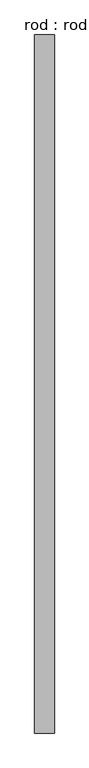
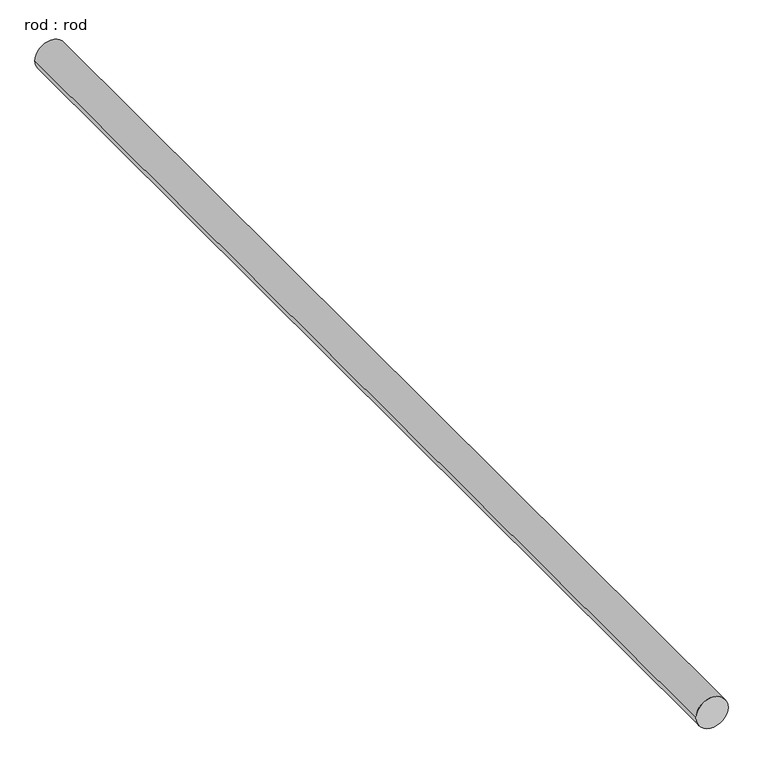
"""IFC4 building model written with IfcOpenShell, lengths in millimetres: proxy geometry, rod : rod."""

import ifcopenshell
import ifcopenshell.guid

model = None  # the IFC model being written
_history = None  # IfcOwnerHistory: only IFC2X3 demands one
_inside = {}  # id of a spatial element -> (the spatial element, [elements in it])
_under = {}  # id of a project, library or spatial element -> (it, [spatial elements below it])
_declared = {}  # id of a project -> (the project, [libraries it declares])
_typed = {}  # id of a type object -> (the type object, [elements of that type])
_made_of = {}  # id of a material, layer set ... -> (it, [elements and type objects made of it])


def new_model(schema):
    """Start an empty IFC model of exactly this schema.

    Asked for "IFC4X3", IfcOpenShell would pick the latest addendum, in which some entities
    have other attributes; the version numbers below select the first issue.
    IFC2X3 requires an IfcOwnerHistory on every rooted entity: one is made here for all.
    """
    global model, _history
    if schema == "IFC4X3":
        model = ifcopenshell.file(schema_version=(4, 3, 0, 0))
    else:
        model = ifcopenshell.file(schema=schema)
    _inside.clear()
    _under.clear()
    _declared.clear()
    _typed.clear()
    _made_of.clear()
    _history = None
    if model.schema == "IFC2X3":
        org = make("IfcOrganization", Name="unknown")
        user = make(
            "IfcPersonAndOrganization",
            ThePerson=make("IfcPerson", FamilyName="unknown"),
            TheOrganization=org,
        )
        app = make(
            "IfcApplication",
            ApplicationDeveloper=org,
            Version="unknown",
            ApplicationFullName="unknown",
            ApplicationIdentifier="unknown",
        )
        _history = make(
            "IfcOwnerHistory",
            OwningUser=user,
            OwningApplication=app,
            ChangeAction="ADDED",
            CreationDate=0,
        )
    return model


def make(cls, **values):
    """One entity of the class cls with the attributes given. An attribute that is None is left unset."""
    return model.create_entity(
        cls, **{name: value for name, value in values.items() if value is not None}
    )


def rooted(cls, **values):
    """An entity with a GlobalId (a new one), such as an element, a storey or a relation."""
    return make(cls, GlobalId=ifcopenshell.guid.new(), OwnerHistory=_history, **values)


def si_unit(unit_type, name, prefix=None):
    """IfcSIUnit, for example si_unit("LENGTHUNIT", "METRE", prefix="MILLI")."""
    return make("IfcSIUnit", UnitType=unit_type, Prefix=prefix, Name=name)


def assignment(units):
    """IfcUnitAssignment: the units of a project."""
    return None if units is None else make("IfcUnitAssignment", Units=units)


def point(xyz):
    """IfcCartesianPoint."""
    return None if xyz is None else make("IfcCartesianPoint", Coordinates=xyz)


def direction(xyz):
    """IfcDirection."""
    return None if xyz is None else make("IfcDirection", DirectionRatios=xyz)


def frame(location, z_axis=None, x_axis=None):
    """IfcAxis2Placement3D, a coordinate frame: its origin and axes. An axis left out is left unset."""
    return make(
        "IfcAxis2Placement3D",
        Location=point(location),
        Axis=direction(z_axis),
        RefDirection=direction(x_axis),
    )


def frame_2d(location, x_axis=None):
    """IfcAxis2Placement2D, a coordinate frame in the plane: its origin and x axis."""
    return make(
        "IfcAxis2Placement2D", Location=point(location), RefDirection=direction(x_axis)
    )


def origin():
    """The frame at (0, 0, 0) with its axes left unset."""
    return frame((0.0, 0.0, 0.0))


def place(relative_to, where):
    """IfcLocalPlacement: puts the frame where relative to a parent placement (None: the world)."""
    return make(
        "IfcLocalPlacement", PlacementRelTo=relative_to, RelativePlacement=where
    )


def context(
    kind, dimensions, precision=None, world=None, true_north=None, identifier=None
):
    """IfcGeometricRepresentationContext, for example the 3D "Model" context."""
    return make(
        "IfcGeometricRepresentationContext",
        ContextIdentifier=identifier,
        ContextType=kind,
        CoordinateSpaceDimension=dimensions,
        Precision=precision,
        WorldCoordinateSystem=world,
        TrueNorth=true_north,
    )


def project(units=None, contexts=None):
    """IfcProject with its units and contexts."""
    return rooted(
        "IfcProject",
        Name="project",
        RepresentationContexts=contexts,
        UnitsInContext=assignment(units),
    )


def spatial(cls, under=None, at=None, **own):
    """A site, building, storey or space (cls), placed at a placement, below another one or the project."""
    s = rooted(cls, ObjectPlacement=at, **own)
    if under is not None:
        _under.setdefault(under.id(), (under, []))[1].append(s)
    return s


def circle_curve(where, radius):
    """IfcCircle in the frame where."""
    return make("IfcCircle", Position=where, Radius=radius)


def trimmed(basis, trim1, trim2, sense, master):
    """IfcTrimmedCurve: the piece of a basis curve between two trims."""
    return make(
        "IfcTrimmedCurve",
        BasisCurve=basis,
        Trim1=trim1,
        Trim2=trim2,
        SenseAgreement=sense,
        MasterRepresentation=master,
    )


def segment(curve, same_sense, transition):
    """IfcCompositeCurveSegment."""
    return make(
        "IfcCompositeCurveSegment",
        Transition=transition,
        SameSense=same_sense,
        ParentCurve=curve,
    )


def composite_curve(segments, self_intersect=None):
    """IfcCompositeCurve: segments joined end to end."""
    return make("IfcCompositeCurve", Segments=segments, SelfIntersect=self_intersect)


def outline(outer, holes=None, kind="AREA"):
    """IfcArbitraryClosedProfileDef: a profile drawn as a closed curve; with holes, ...WithVoids."""
    if holes is None:
        return make("IfcArbitraryClosedProfileDef", ProfileType=kind, OuterCurve=outer)
    return make(
        "IfcArbitraryProfileDefWithVoids",
        ProfileType=kind,
        OuterCurve=outer,
        InnerCurves=holes,
    )


def extrude(swept, where, along, depth):
    """IfcExtrudedAreaSolid: the profile swept, set in the frame where, extruded along a direction by depth."""
    return make(
        "IfcExtrudedAreaSolid",
        SweptArea=swept,
        Position=where,
        ExtrudedDirection=direction(along),
        Depth=depth,
    )


def shape(context_of_items, identifier, shape_type, items):
    """IfcShapeRepresentation: the items that make up one representation, for example the "Body"."""
    return make(
        "IfcShapeRepresentation",
        ContextOfItems=context_of_items,
        RepresentationIdentifier=identifier,
        RepresentationType=shape_type,
        Items=items,
    )


def source(mapping_origin, context_of_items, identifier, shape_type, items):
    """IfcRepresentationMap: a shape defined once, which mapped items show again and again."""
    return make(
        "IfcRepresentationMap",
        MappingOrigin=mapping_origin,
        MappedRepresentation=shape(context_of_items, identifier, shape_type, items),
    )


def transform(
    local_origin,
    x_axis=None,
    y_axis=None,
    z_axis=None,
    scale=None,
    scale2=None,
    scale3=None,
    uniform=True,
):
    """IfcCartesianTransformationOperator3D, or its non-uniform kind. x_axis, y_axis, z_axis: its Axis1, 2, 3."""
    if uniform:
        return make(
            "IfcCartesianTransformationOperator3D",
            Axis1=direction(x_axis),
            Axis2=direction(y_axis),
            LocalOrigin=point(local_origin),
            Scale=scale,
            Axis3=direction(z_axis),
        )
    return make(
        "IfcCartesianTransformationOperator3DnonUniform",
        Axis1=direction(x_axis),
        Axis2=direction(y_axis),
        LocalOrigin=point(local_origin),
        Scale=scale,
        Axis3=direction(z_axis),
        Scale2=scale2,
        Scale3=scale3,
    )


def mapped(mapping_source, mapping_target):
    """IfcMappedItem: shows the shape of a source again, moved by a transform."""
    return make(
        "IfcMappedItem", MappingSource=mapping_source, MappingTarget=mapping_target
    )


def made_of(thing, what):
    """Note that an element or type object is made of a material, layer set ...; save() writes the relation."""
    if what is not None:
        _made_of.setdefault(what.id(), (what, []))[1].append(thing)
    return thing


def element(
    cls,
    number,
    at=None,
    inside=None,
    cuts=None,
    type_object=None,
    material=None,
    context=None,
    identifier="Body",
    shape_type=None,
    held_by="IfcProductDefinitionShape",
    body=None,
    shapes=None,
    **own,
):
    """One element of the class cls, such as IfcWall. Its Tag is "e" and its number.

    at: its placement. inside: the storey or other place that contains it. cuts: it is an
    opening in that element (IfcRelVoidsElement). A single representation is given by context,
    identifier, shape_type and body (its items); several are given by shapes. held_by: the class
    of the entity that holds the representations. save() writes the other relations.
    """
    e = rooted(cls, Tag="e%d" % number, ObjectPlacement=at, **own)
    if body is not None:
        shapes = [shape(context, identifier, shape_type, body)]
    if shapes is not None:
        e.Representation = make(held_by, Representations=shapes)
    if inside is not None:
        _inside.setdefault(inside.id(), (inside, []))[1].append(e)
    if cuts is not None:
        rooted(
            "IfcRelVoidsElement", RelatingBuildingElement=cuts, RelatedOpeningElement=e
        )
    if type_object is not None:
        _typed.setdefault(type_object.id(), (type_object, []))[1].append(e)
    return made_of(e, material)


def aggregate(whole, parts):
    """IfcRelAggregates: a whole, such as a stair, and the parts it consists of."""
    return rooted("IfcRelAggregates", RelatingObject=whole, RelatedObjects=parts)


def save(model, path):
    """Write the relations noted so far, then the file.

    IfcRelAggregates (storeys below a building ...), IfcRelContainedInSpatialStructure (elements
    in a storey), IfcRelDefinesByType, IfcRelAssociatesMaterial and IfcRelDeclares: one each for
    every whole, place, type object, material and project.
    """
    for whole, parts in _under.values():
        aggregate(whole, parts)
    for where, things in _inside.values():
        rooted(
            "IfcRelContainedInSpatialStructure",
            RelatedElements=things,
            RelatingStructure=where,
        )
    for kind, things in _typed.values():
        rooted("IfcRelDefinesByType", RelatedObjects=things, RelatingType=kind)
    for what, things in _made_of.values():
        rooted("IfcRelAssociatesMaterial", RelatedObjects=things, RelatingMaterial=what)
    for by, libraries in _declared.values():
        rooted("IfcRelDeclares", RelatingContext=by, RelatedDefinitions=libraries)
    model.write(path)


def rod_rod_25347198(model_context):
    return source(origin(), model_context, "Body", "SweptSolid", [
        extrude(outline(composite_curve([segment(trimmed(circle_curve(frame_2d((0.0108462, 0.0)), 200.0), [point((0.0108462, 200.0))], [point((0.0108462, -200.0))], False, "CARTESIAN"), True, "CONTINUOUS"), segment(trimmed(circle_curve(frame_2d((0.0108462, 0.0)), 200.0), [point((0.0108462, -200.0))], [point((0.0108462, 200.0))], False, "CARTESIAN"), True, "CONTINUOUS")], self_intersect=False)), frame((0.0, -3032.2713847, 0.0), z_axis=(0.0, 1.0, 0.0), x_axis=(0.0, 0.0, 1.0)), (0.0, 0.0, 1.0), 14250.0),
    ])


if __name__ == "__main__":
    model = new_model("IFC4")
    model_context = context("Model", 3, world=origin())
    ifc_project = project(units=[si_unit("LENGTHUNIT", "METRE", prefix="MILLI")], contexts=[model_context])
    site = spatial("IfcSite", under=ifc_project)
    building = spatial("IfcBuilding", under=site)
    placement = place(None, origin())
    rod_rod_shape = rod_rod_25347198(model_context)
    element("IfcBuildingElementProxy", 1, Name="rod : rod", ObjectType="rod : rod", at=placement, inside=building, context=model_context, shape_type="MappedRepresentation", body=[
        mapped(rod_rod_shape, transform((0.0, 0.0, 0.0), x_axis=(1.0, 0.0, 0.0), y_axis=(0.0, 1.0, 0.0), z_axis=(0.0, 0.0, 1.0))),
    ])
    save(model, "model.ifc")

# Revit data of these elements
# Type "rod : rod"
#   Default Elevation = 0
